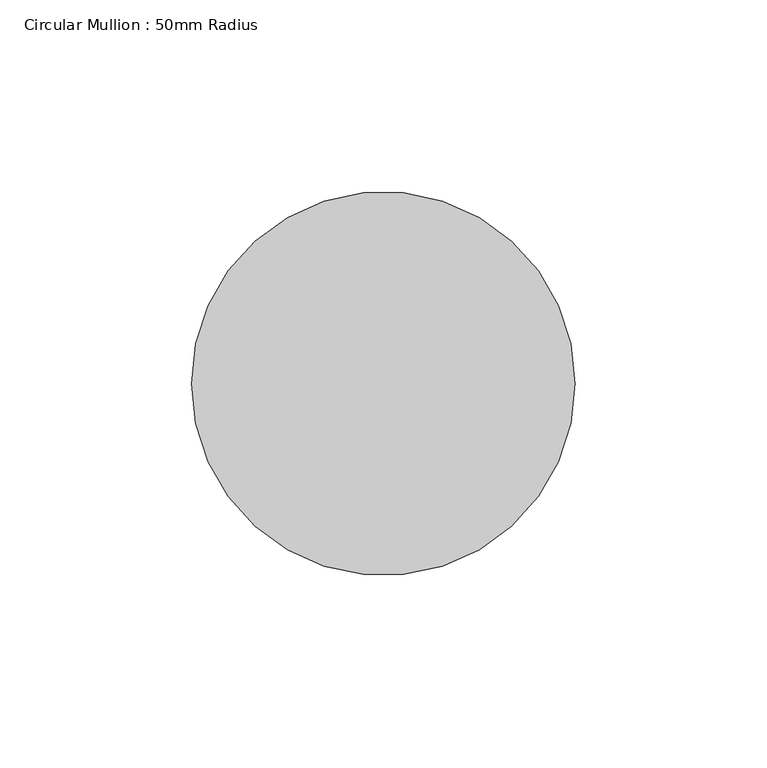
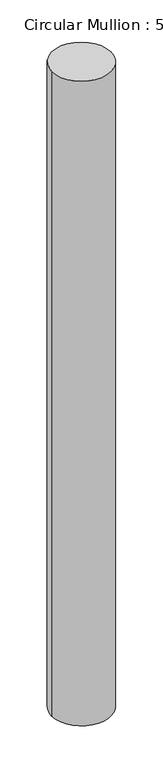
"""IFC4 building model written with IfcOpenShell, lengths in millimetres: member geometry, Circular Mullion : 50mm Radius."""

from ifc_helpers import new_model, si_unit, point, frame, origin, origin_2d, place, context, project, spatial, circle_curve, trimmed, segment, composite_curve, outline, extrude, source, transform, mapped, element, save


def circular_mullion_50mm_radius_187899ec(model_context):
    return source(origin(), model_context, "Body", "SweptSolid", [
        extrude(outline(composite_curve([segment(trimmed(circle_curve(origin_2d(), 50.0), [point((50.0, 0.0))], [point((-50.0, 0.0))], False, "CARTESIAN"), True, "CONTINUOUS"), segment(trimmed(circle_curve(origin_2d(), 50.0), [point((-50.0, 0.0))], [point((50.0, 0.0))], False, "CARTESIAN"), True, "CONTINUOUS")], self_intersect=False)), frame((0.0, 0.0, -1151.9848729), z_axis=(0.0, 0.0, 1.0), x_axis=(1.0, 0.0, 0.0)), (0.0, 0.0, 1.0), 1151.9848729),
    ])


if __name__ == "__main__":
    model = new_model("IFC4")
    model_context = context("Model", 3, world=origin())
    ifc_project = project(units=[si_unit("LENGTHUNIT", "METRE", prefix="MILLI")], contexts=[model_context])
    site = spatial("IfcSite", under=ifc_project)
    building = spatial("IfcBuilding", under=site)
    placement = place(None, origin())
    circular_mullion_50mm_radius_shape = circular_mullion_50mm_radius_187899ec(model_context)
    element("IfcMember", 1, ObjectType="Circular Mullion : 50mm Radius", at=placement, inside=building, context=model_context, shape_type="MappedRepresentation", body=[
        mapped(circular_mullion_50mm_radius_shape, transform((0.0, 0.0, 0.0), x_axis=(1.0, 0.0, 0.0), y_axis=(0.0, 1.0, 0.0), z_axis=(0.0, 0.0, 1.0))),
    ])
    save(model, "model.ifc")

# Revit data of these elements
# Type "Circular Mullion : 50mm Radius"
#   built-in parameter 1007350 = 0.164042 (stored number, unit not read)
# Element 1 (IfcMember, "Circular Mullion : 50mm Radius")
#   Materials on its faces: "Aluminium"
# Materials
#   "Aluminium": class "Metal", colour RGB 247 247 247, transparency 0, Description = "Aluminium 6061", Cost = 0
